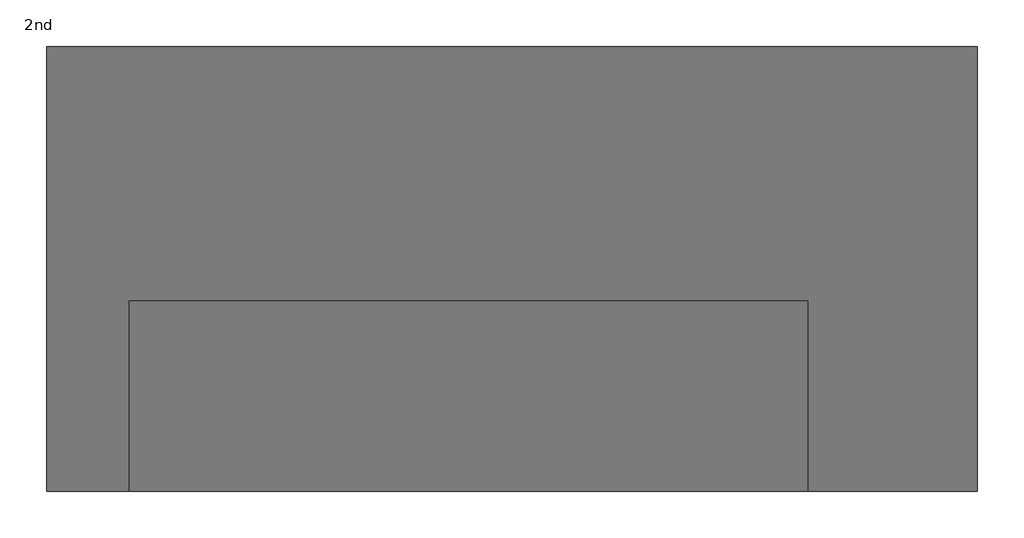
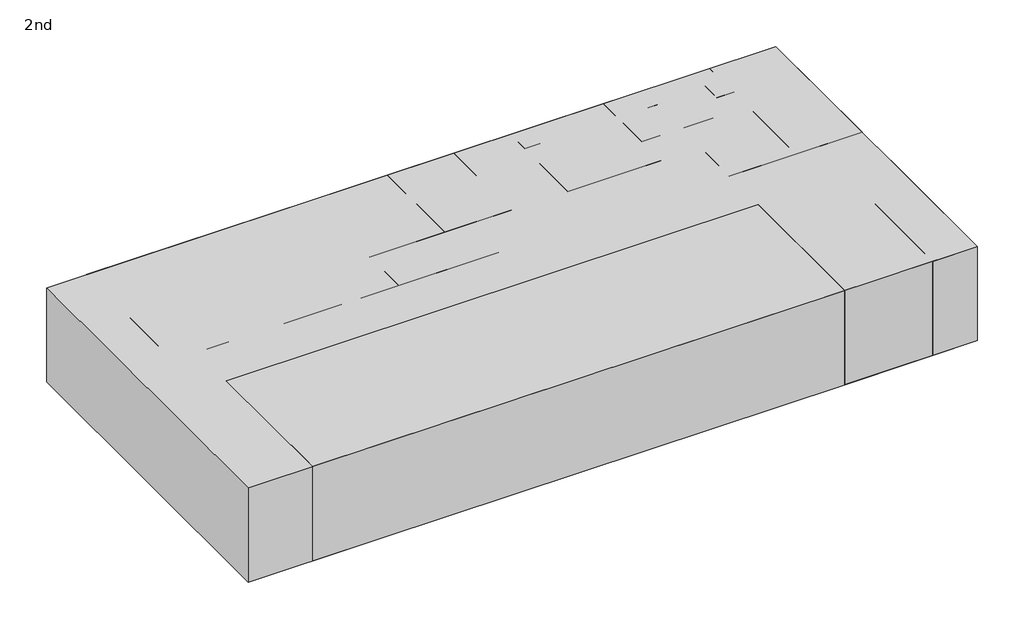
# One storey: 17 proxies.
"""IFC4 building model written with IfcOpenShell, lengths in millimetres."""

import ifcopenshell
import ifcopenshell.guid

model = None  # the IFC model being written
_history = None  # IfcOwnerHistory: only IFC2X3 demands one
_inside = {}  # id of a spatial element -> (the spatial element, [elements in it])
_under = {}  # id of a project, library or spatial element -> (it, [spatial elements below it])
_declared = {}  # id of a project -> (the project, [libraries it declares])
_typed = {}  # id of a type object -> (the type object, [elements of that type])
_made_of = {}  # id of a material, layer set ... -> (it, [elements and type objects made of it])


def new_model(schema):
    """Start an empty IFC model of exactly this schema.

    Asked for "IFC4X3", IfcOpenShell would pick the latest addendum, in which some entities
    have other attributes; the version numbers below select the first issue.
    IFC2X3 requires an IfcOwnerHistory on every rooted entity: one is made here for all.
    """
    global model, _history
    if schema == "IFC4X3":
        model = ifcopenshell.file(schema_version=(4, 3, 0, 0))
    else:
        model = ifcopenshell.file(schema=schema)
    _inside.clear()
    _under.clear()
    _declared.clear()
    _typed.clear()
    _made_of.clear()
    _history = None
    if model.schema == "IFC2X3":
        org = make("IfcOrganization", Name="unknown")
        user = make(
            "IfcPersonAndOrganization",
            ThePerson=make("IfcPerson", FamilyName="unknown"),
            TheOrganization=org,
        )
        app = make(
            "IfcApplication",
            ApplicationDeveloper=org,
            Version="unknown",
            ApplicationFullName="unknown",
            ApplicationIdentifier="unknown",
        )
        _history = make(
            "IfcOwnerHistory",
            OwningUser=user,
            OwningApplication=app,
            ChangeAction="ADDED",
            CreationDate=0,
        )
    return model


def make(cls, **values):
    """One entity of the class cls with the attributes given. An attribute that is None is left unset."""
    return model.create_entity(
        cls, **{name: value for name, value in values.items() if value is not None}
    )


def rooted(cls, **values):
    """An entity with a GlobalId (a new one), such as an element, a storey or a relation."""
    return make(cls, GlobalId=ifcopenshell.guid.new(), OwnerHistory=_history, **values)


def si_unit(unit_type, name, prefix=None):
    """IfcSIUnit, for example si_unit("LENGTHUNIT", "METRE", prefix="MILLI")."""
    return make("IfcSIUnit", UnitType=unit_type, Prefix=prefix, Name=name)


def assignment(units):
    """IfcUnitAssignment: the units of a project."""
    return None if units is None else make("IfcUnitAssignment", Units=units)


def point(xyz):
    """IfcCartesianPoint."""
    return None if xyz is None else make("IfcCartesianPoint", Coordinates=xyz)


def direction(xyz):
    """IfcDirection."""
    return None if xyz is None else make("IfcDirection", DirectionRatios=xyz)


def frame(location, z_axis=None, x_axis=None):
    """IfcAxis2Placement3D, a coordinate frame: its origin and axes. An axis left out is left unset."""
    return make(
        "IfcAxis2Placement3D",
        Location=point(location),
        Axis=direction(z_axis),
        RefDirection=direction(x_axis),
    )


def origin():
    """The frame at (0, 0, 0) with its axes left unset."""
    return frame((0.0, 0.0, 0.0))


def origin_with_axes():
    """The frame at (0, 0, 0) with the z axis (0, 0, 1) and the x axis (1, 0, 0) written out."""
    return frame((0.0, 0.0, 0.0), z_axis=(0.0, 0.0, 1.0), x_axis=(1.0, 0.0, 0.0))


def place(relative_to, where):
    """IfcLocalPlacement: puts the frame where relative to a parent placement (None: the world)."""
    return make(
        "IfcLocalPlacement", PlacementRelTo=relative_to, RelativePlacement=where
    )


def context(
    kind, dimensions, precision=None, world=None, true_north=None, identifier=None
):
    """IfcGeometricRepresentationContext, for example the 3D "Model" context."""
    return make(
        "IfcGeometricRepresentationContext",
        ContextIdentifier=identifier,
        ContextType=kind,
        CoordinateSpaceDimension=dimensions,
        Precision=precision,
        WorldCoordinateSystem=world,
        TrueNorth=true_north,
    )


def project(units=None, contexts=None):
    """IfcProject with its units and contexts."""
    return rooted(
        "IfcProject",
        Name="project",
        RepresentationContexts=contexts,
        UnitsInContext=assignment(units),
    )


def spatial(cls, under=None, at=None, **own):
    """A site, building, storey or space (cls), placed at a placement, below another one or the project."""
    s = rooted(cls, ObjectPlacement=at, **own)
    if under is not None:
        _under.setdefault(under.id(), (under, []))[1].append(s)
    return s


def polyline(points):
    """IfcPolyline through the points."""
    return make("IfcPolyline", Points=[point(p) for p in points])


def outline(outer, holes=None, kind="AREA"):
    """IfcArbitraryClosedProfileDef: a profile drawn as a closed curve; with holes, ...WithVoids."""
    if holes is None:
        return make("IfcArbitraryClosedProfileDef", ProfileType=kind, OuterCurve=outer)
    return make(
        "IfcArbitraryProfileDefWithVoids",
        ProfileType=kind,
        OuterCurve=outer,
        InnerCurves=holes,
    )


def extrude(swept, where, along, depth):
    """IfcExtrudedAreaSolid: the profile swept, set in the frame where, extruded along a direction by depth."""
    return make(
        "IfcExtrudedAreaSolid",
        SweptArea=swept,
        Position=where,
        ExtrudedDirection=direction(along),
        Depth=depth,
    )


def shape(context_of_items, identifier, shape_type, items):
    """IfcShapeRepresentation: the items that make up one representation, for example the "Body"."""
    return make(
        "IfcShapeRepresentation",
        ContextOfItems=context_of_items,
        RepresentationIdentifier=identifier,
        RepresentationType=shape_type,
        Items=items,
    )


def source(mapping_origin, context_of_items, identifier, shape_type, items):
    """IfcRepresentationMap: a shape defined once, which mapped items show again and again."""
    return make(
        "IfcRepresentationMap",
        MappingOrigin=mapping_origin,
        MappedRepresentation=shape(context_of_items, identifier, shape_type, items),
    )


def transform(
    local_origin,
    x_axis=None,
    y_axis=None,
    z_axis=None,
    scale=None,
    scale2=None,
    scale3=None,
    uniform=True,
):
    """IfcCartesianTransformationOperator3D, or its non-uniform kind. x_axis, y_axis, z_axis: its Axis1, 2, 3."""
    if uniform:
        return make(
            "IfcCartesianTransformationOperator3D",
            Axis1=direction(x_axis),
            Axis2=direction(y_axis),
            LocalOrigin=point(local_origin),
            Scale=scale,
            Axis3=direction(z_axis),
        )
    return make(
        "IfcCartesianTransformationOperator3DnonUniform",
        Axis1=direction(x_axis),
        Axis2=direction(y_axis),
        LocalOrigin=point(local_origin),
        Scale=scale,
        Axis3=direction(z_axis),
        Scale2=scale2,
        Scale3=scale3,
    )


def mapped(mapping_source, mapping_target):
    """IfcMappedItem: shows the shape of a source again, moved by a transform."""
    return make(
        "IfcMappedItem", MappingSource=mapping_source, MappingTarget=mapping_target
    )


def made_of(thing, what):
    """Note that an element or type object is made of a material, layer set ...; save() writes the relation."""
    if what is not None:
        _made_of.setdefault(what.id(), (what, []))[1].append(thing)
    return thing


def element(
    cls,
    number,
    at=None,
    inside=None,
    cuts=None,
    type_object=None,
    material=None,
    context=None,
    identifier="Body",
    shape_type=None,
    held_by="IfcProductDefinitionShape",
    body=None,
    shapes=None,
    **own,
):
    """One element of the class cls, such as IfcWall. Its Tag is "e" and its number.

    at: its placement. inside: the storey or other place that contains it. cuts: it is an
    opening in that element (IfcRelVoidsElement). A single representation is given by context,
    identifier, shape_type and body (its items); several are given by shapes. held_by: the class
    of the entity that holds the representations. save() writes the other relations.
    """
    e = rooted(cls, Tag="e%d" % number, ObjectPlacement=at, **own)
    if body is not None:
        shapes = [shape(context, identifier, shape_type, body)]
    if shapes is not None:
        e.Representation = make(held_by, Representations=shapes)
    if inside is not None:
        _inside.setdefault(inside.id(), (inside, []))[1].append(e)
    if cuts is not None:
        rooted(
            "IfcRelVoidsElement", RelatingBuildingElement=cuts, RelatedOpeningElement=e
        )
    if type_object is not None:
        _typed.setdefault(type_object.id(), (type_object, []))[1].append(e)
    return made_of(e, material)


def aggregate(whole, parts):
    """IfcRelAggregates: a whole, such as a stair, and the parts it consists of."""
    return rooted("IfcRelAggregates", RelatingObject=whole, RelatedObjects=parts)


def save(model, path):
    """Write the relations noted so far, then the file.

    IfcRelAggregates (storeys below a building ...), IfcRelContainedInSpatialStructure (elements
    in a storey), IfcRelDefinesByType, IfcRelAssociatesMaterial and IfcRelDeclares: one each for
    every whole, place, type object, material and project.
    """
    for whole, parts in _under.values():
        aggregate(whole, parts)
    for where, things in _inside.values():
        rooted(
            "IfcRelContainedInSpatialStructure",
            RelatedElements=things,
            RelatingStructure=where,
        )
    for kind, things in _typed.values():
        rooted("IfcRelDefinesByType", RelatedObjects=things, RelatingType=kind)
    for what, things in _made_of.values():
        rooted("IfcRelAssociatesMaterial", RelatedObjects=things, RelatingMaterial=what)
    for by, libraries in _declared.values():
        rooted("IfcRelDeclares", RelatingContext=by, RelatedDefinitions=libraries)
    model.write(path)


def generic_models_29bcd6f9(model_context):
    return source(origin(), model_context, "Body", "SweptSolid", [
        extrude(outline(polyline([(2000.0, 4500.0), (2000.0, -4500.0), (-2000.0, -4500.0), (-2000.0, 4500.0), (2000.0, 4500.0)])), origin_with_axes(), (0.0, 0.0, 1.0), 6000.0),
    ])


def generic_models_5634f436(model_context):
    return source(origin(), model_context, "Body", "SweptSolid", [
        extrude(outline(polyline([(1350.0, 3000.0), (1350.0, -3000.0), (-1350.0, -3000.0), (-1350.0, 3000.0), (1350.0, 3000.0)])), origin_with_axes(), (0.0, 0.0, 1.0), 6000.0),
    ])


def generic_models_71e2440f(model_context):
    return source(origin(), model_context, "Body", "SweptSolid", [
        extrude(outline(polyline([(500.0, 1250.0), (500.0, -1250.0), (-500.0, -1250.0), (-500.0, 1250.0), (500.0, 1250.0)])), origin_with_axes(), (0.0, 0.0, 1.0), 6000.0),
    ])


def generic_models_57c7875f(model_context):
    return source(origin(), model_context, "Body", "SweptSolid", [
        extrude(outline(polyline([(4500.0, 16000.0), (4500.0, -16000.0), (-4500.0, -16000.0), (-4500.0, 16000.0), (4500.0, 16000.0)])), origin_with_axes(), (0.0, 0.0, 1.0), 6000.0),
    ])


def generic_models_7bff30ad(model_context):
    return source(origin(), model_context, "Body", "SweptSolid", [
        extrude(outline(polyline([(2000.0, 2000.0), (2000.0, -2000.0), (-2000.0, -2000.0), (-2000.0, 2000.0), (2000.0, 2000.0)])), origin_with_axes(), (0.0, 0.0, 1.0), 6000.0),
    ])


def generic_models_5b7b272c(model_context):
    return source(origin(), model_context, "Body", "SweptSolid", [
        extrude(outline(polyline([(2000.0, 2500.0), (2000.0, -2500.0), (-2000.0, -2500.0), (-2000.0, 2500.0), (2000.0, 2500.0)])), origin_with_axes(), (0.0, 0.0, 1.0), 6000.0),
    ])


def generic_models_47b98be1(model_context):
    return source(origin(), model_context, "Body", "SweptSolid", [
        extrude(outline(polyline([(1200.0, 2000.0), (1200.0, -2000.0), (-1200.0, -2000.0), (-1200.0, 2000.0), (1200.0, 2000.0)])), origin_with_axes(), (0.0, 0.0, 1.0), 6000.0),
    ])


def generic_models_7a053eeb(model_context):
    return source(origin(), model_context, "Body", "SweptSolid", [
        extrude(outline(polyline([(1200.0, 750.0), (1200.0, -750.0), (-1200.0, -750.0), (-1200.0, 750.0), (1200.0, 750.0)])), origin_with_axes(), (0.0, 0.0, 1.0), 6000.0),
    ])


def generic_models_ec17d728(model_context):
    return source(origin(), model_context, "Body", "SweptSolid", [
        extrude(outline(polyline([(2800.0, 3000.0), (2800.0, -3000.0), (-2800.0, -3000.0), (-2800.0, 3000.0), (2800.0, 3000.0)])), origin_with_axes(), (0.0, 0.0, 1.0), 6000.0),
    ])


def generic_models_85897e09(model_context):
    return source(origin(), model_context, "Body", "SweptSolid", [
        extrude(outline(polyline([(2800.0, 750.0), (2800.0, -750.0), (-2800.0, -750.0), (-2800.0, 750.0), (2800.0, 750.0)])), origin_with_axes(), (0.0, 0.0, 1.0), 6000.0),
    ])


def generic_models_b79df083(model_context):
    return source(origin(), model_context, "Body", "SweptSolid", [
        extrude(outline(polyline([(4500.0, 4500.0), (4500.0, -4500.0), (-4500.0, -4500.0), (-4500.0, 4500.0), (4500.0, 4500.0)])), origin_with_axes(), (0.0, 0.0, 1.0), 6000.0),
    ])


def generic_models_98b71764(model_context):
    return source(origin(), model_context, "Body", "SweptSolid", [
        extrude(outline(polyline([(2000.0, 3000.0), (2000.0, -3000.0), (-2000.0, -3000.0), (-2000.0, 3000.0), (2000.0, 3000.0)])), origin_with_axes(), (0.0, 0.0, 1.0), 6000.0),
    ])


def generic_models_8af91fed(model_context):
    return source(origin(), model_context, "Body", "SweptSolid", [
        extrude(outline(polyline([(2250.0, 3000.0), (2250.0, -3000.0), (-2250.0, -3000.0), (-2250.0, 3000.0), (2250.0, 3000.0)])), origin_with_axes(), (0.0, 0.0, 1.0), 6000.0),
    ])


def generic_models_542cc789(model_context):
    return source(origin(), model_context, "Body", "SweptSolid", [
        extrude(outline(polyline([(1500.0, 3000.0), (1500.0, -3000.0), (-1500.0, -3000.0), (-1500.0, 3000.0), (1500.0, 3000.0)])), origin_with_axes(), (0.0, 0.0, 1.0), 6000.0),
    ])


def generic_models_af0009da(model_context):
    return source(origin(), model_context, "Body", "SweptSolid", [
        extrude(outline(polyline([(4500.0, 6800.0), (4500.0, -6800.0), (-4500.0, -6800.0), (-4500.0, 6800.0), (4500.0, 6800.0)])), origin_with_axes(), (0.0, 0.0, 1.0), 6000.0),
    ])


def generic_models_4d084078(model_context):
    return source(origin(), model_context, "Body", "SweptSolid", [
        extrude(outline(polyline([(4000.0, 4500.0), (4000.0, -4500.0), (-4000.0, -4500.0), (-4000.0, 4500.0), (4000.0, 4500.0)])), origin_with_axes(), (0.0, 0.0, 1.0), 6000.0),
    ])


def generic_models_b3b0fa1d(model_context):
    return source(origin(), model_context, "Body", "SweptSolid", [
        extrude(outline(polyline([(21950.0, 10500.0), (21950.0, -10500.0), (-21950.0, -10500.0), (-21950.0, 10500.0), (21950.0, 10500.0)])), origin_with_axes(), (0.0, 0.0, 1.0), 6000.0),
    ])


model = new_model("IFC4")

# Units and contexts
model_context = context("Model", 3, world=origin())
ifc_project = project(units=[si_unit("LENGTHUNIT", "METRE", prefix="MILLI")], contexts=[model_context])

# Site, building, storey
site = spatial("IfcSite", under=ifc_project)
building = spatial("IfcBuilding", under=site)
storey = spatial("IfcBuildingStorey", under=building, Name="2nd", Elevation=14000.0)

# Proxies
placement = place(None, origin())
generic_models_shape = generic_models_29bcd6f9(model_context)
element("IfcBuildingElementProxy", 1, Name="Space Planning Box_hec : Space Planning Box_hec", ObjectType="Space Planning Box_hec : Space Planning Box_hec", at=placement, inside=storey, context=model_context, shape_type="MappedRepresentation", body=[
    mapped(generic_models_shape, transform((198014.1020501, 147515.7581198, 14000.0), x_axis=(1.0, 0.0, 0.0), y_axis=(0.0, 1.0, 0.0), z_axis=(0.0, 0.0, 1.0))),
])
generic_models_2_shape = generic_models_5634f436(model_context)
element("IfcBuildingElementProxy", 2, Name="Space Planning Box_hec : Space Planning Box_hec", ObjectType="Space Planning Box_hec : Space Planning Box_hec", at=placement, inside=storey, context=model_context, shape_type="MappedRepresentation", body=[
    mapped(generic_models_2_shape, transform((198664.1020501, 134015.7581198, 14000.0), x_axis=(1.0, 0.0, 0.0), y_axis=(0.0, 1.0, 0.0), z_axis=(0.0, 0.0, 1.0))),
])
generic_models_3_shape = generic_models_71e2440f(model_context)
element("IfcBuildingElementProxy", 3, Name="Space Planning Box_hec : Space Planning Box_hec", ObjectType="Space Planning Box_hec : Space Planning Box_hec", at=placement, inside=storey, context=model_context, shape_type="MappedRepresentation", body=[
    mapped(generic_models_3_shape, transform((195514.1020501, 150765.7581198, 14000.0), x_axis=(1.0, 0.0, 0.0), y_axis=(0.0, 1.0, 0.0), z_axis=(0.0, 0.0, 1.0))),
])
generic_models_4_shape = generic_models_57c7875f(model_context)
element("IfcBuildingElementProxy", 4, Name="Space Planning Box_hec : Space Planning Box_hec", ObjectType="Space Planning Box_hec : Space Planning Box_hec", at=placement, inside=storey, context=model_context, shape_type="MappedRepresentation", body=[
    mapped(generic_models_4_shape, transform((176014.1020501, 135515.7581198, 14000.0), x_axis=(0.0, -1.0, 0.0), y_axis=(1.0, 0.0, 0.0), z_axis=(0.0, 0.0, 1.0))),
])
generic_models_5_shape = generic_models_7bff30ad(model_context)
element("IfcBuildingElementProxy", 5, Name="Space Planning Box_hec : Space Planning Box_hec", ObjectType="Space Planning Box_hec : Space Planning Box_hec", at=placement, inside=storey, context=model_context, shape_type="MappedRepresentation", body=[
    mapped(generic_models_5_shape, transform((194014.1020501, 150015.7581198, 14000.0), x_axis=(1.0, 0.0, 0.0), y_axis=(0.0, 1.0, 0.0), z_axis=(0.0, 0.0, 1.0))),
])
generic_models_6_shape = generic_models_5b7b272c(model_context)
element("IfcBuildingElementProxy", 6, Name="Space Planning Box_hec : Space Planning Box_hec", ObjectType="Space Planning Box_hec : Space Planning Box_hec", at=placement, inside=storey, context=model_context, shape_type="MappedRepresentation", body=[
    mapped(generic_models_6_shape, transform((194014.1020501, 145515.7581198, 14000.0), x_axis=(1.0, 0.0, 0.0), y_axis=(0.0, 1.0, 0.0), z_axis=(0.0, 0.0, 1.0))),
])
generic_models_7_shape = generic_models_47b98be1(model_context)
element("IfcBuildingElementProxy", 7, Name="Space Planning Box_hec : Space Planning Box_hec", ObjectType="Space Planning Box_hec : Space Planning Box_hec", at=placement, inside=storey, context=model_context, shape_type="MappedRepresentation", body=[
    mapped(generic_models_7_shape, transform((190814.1020501, 150015.7581198, 14000.0), x_axis=(1.0, 0.0, 0.0), y_axis=(0.0, 1.0, 0.0), z_axis=(0.0, 0.0, 1.0))),
])
generic_models_8_shape = generic_models_7a053eeb(model_context)
element("IfcBuildingElementProxy", 8, Name="Space Planning Box_hec : Space Planning Box_hec", ObjectType="Space Planning Box_hec : Space Planning Box_hec", at=placement, inside=storey, context=model_context, shape_type="MappedRepresentation", body=[
    mapped(generic_models_8_shape, transform((190814.1020501, 151265.7581198, 14000.0), x_axis=(1.0, 0.0, 0.0), y_axis=(0.0, 1.0, 0.0), z_axis=(0.0, 0.0, 1.0))),
])
generic_models_9_shape = generic_models_ec17d728(model_context)
element("IfcBuildingElementProxy", 9, Name="Space Planning Box_hec : Space Planning Box_hec", ObjectType="Space Planning Box_hec : Space Planning Box_hec", at=placement, inside=storey, context=model_context, shape_type="MappedRepresentation", body=[
    mapped(generic_models_9_shape, transform((186814.1020501, 149015.7581198, 14000.0), x_axis=(1.0, 0.0, 0.0), y_axis=(0.0, 1.0, 0.0), z_axis=(0.0, 0.0, 1.0))),
])
generic_models_10_shape = generic_models_85897e09(model_context)
element("IfcBuildingElementProxy", 10, Name="Space Planning Box_hec : Space Planning Box_hec", ObjectType="Space Planning Box_hec : Space Planning Box_hec", at=placement, inside=storey, context=model_context, shape_type="MappedRepresentation", body=[
    mapped(generic_models_10_shape, transform((186814.1020501, 151265.7581198, 14000.0), x_axis=(1.0, 0.0, 0.0), y_axis=(0.0, 1.0, 0.0), z_axis=(0.0, 0.0, 1.0))),
])
generic_models_11_shape = generic_models_b79df083(model_context)
element("IfcBuildingElementProxy", 11, Name="Space Planning Box_hec : Space Planning Box_hec", ObjectType="Space Planning Box_hec : Space Planning Box_hec", at=placement, inside=storey, context=model_context, shape_type="MappedRepresentation", body=[
    mapped(generic_models_11_shape, transform((185114.1020501, 147515.7581198, 14000.0), x_axis=(1.0, 0.0, 0.0), y_axis=(0.0, 1.0, 0.0), z_axis=(0.0, 0.0, 1.0))),
])
generic_models_12_shape = generic_models_98b71764(model_context)
element("IfcBuildingElementProxy", 12, Name="Space Planning Box_hec : Space Planning Box_hec", ObjectType="Space Planning Box_hec : Space Planning Box_hec", at=placement, inside=storey, context=model_context, shape_type="MappedRepresentation", body=[
    mapped(generic_models_12_shape, transform((178614.1020501, 149015.7581198, 14000.0), x_axis=(1.0, 0.0, 0.0), y_axis=(0.0, 1.0, 0.0), z_axis=(0.0, 0.0, 1.0))),
])
generic_models_13_shape = generic_models_8af91fed(model_context)
element("IfcBuildingElementProxy", 13, Name="Space Planning Box_hec : Space Planning Box_hec", ObjectType="Space Planning Box_hec : Space Planning Box_hec", at=placement, inside=storey, context=model_context, shape_type="MappedRepresentation", body=[
    mapped(generic_models_13_shape, transform((174364.1020501, 149015.7581198, 14000.0), x_axis=(1.0, 0.0, 0.0), y_axis=(0.0, 1.0, 0.0), z_axis=(0.0, 0.0, 1.0))),
])
generic_models_14_shape = generic_models_542cc789(model_context)
element("IfcBuildingElementProxy", 14, Name="Space Planning Box_hec : Space Planning Box_hec", ObjectType="Space Planning Box_hec : Space Planning Box_hec", at=placement, inside=storey, context=model_context, shape_type="MappedRepresentation", body=[
    mapped(generic_models_14_shape, transform((175114.1020501, 144515.7581198, 14000.0), x_axis=(0.0, 1.0, 0.0), y_axis=(-1.0, 0.0, 0.0), z_axis=(0.0, 0.0, 1.0))),
])
generic_models_15_shape = generic_models_af0009da(model_context)
element("IfcBuildingElementProxy", 15, Name="Space Planning Box_hec : Space Planning Box_hec", ObjectType="Space Planning Box_hec : Space Planning Box_hec", at=placement, inside=storey, context=model_context, shape_type="MappedRepresentation", body=[
    mapped(generic_models_15_shape, transform((165314.1020501, 147515.7581198, 14000.0), x_axis=(0.0, -1.0, 0.0), y_axis=(1.0, 0.0, 0.0), z_axis=(0.0, 0.0, 1.0))),
])
generic_models_16_shape = generic_models_4d084078(model_context)
element("IfcBuildingElementProxy", 16, Name="Space Planning Box_hec : Space Planning Box_hec", ObjectType="Space Planning Box_hec : Space Planning Box_hec", at=placement, inside=storey, context=model_context, shape_type="MappedRepresentation", body=[
    mapped(generic_models_16_shape, transform((196014.1020501, 135515.7581198, 14000.0), x_axis=(1.0, 0.0, 0.0), y_axis=(0.0, 1.0, 0.0), z_axis=(0.0, 0.0, 1.0))),
])
generic_models_17_shape = generic_models_b3b0fa1d(model_context)
element("IfcBuildingElementProxy", 17, Name="Space Planning Box_hec : Space Planning Box_hec", ObjectType="Space Planning Box_hec : Space Planning Box_hec", at=placement, inside=storey, context=model_context, shape_type="MappedRepresentation", body=[
    mapped(generic_models_17_shape, transform((178064.1020501, 141515.7581198, 14000.0), x_axis=(1.0, 0.0, 0.0), y_axis=(0.0, 1.0, 0.0), z_axis=(0.0, 0.0, 1.0))),
])

save(model, "model.ifc")

# Revit data of these elements
# Type "Space Planning Box_hec : Space Planning Box_hec"
#   Type Comments = "..."
#   Room Name [instance default] = "?"
#   Interior Finish [instance default] = ""
#   Exterior Finish [instance default] = ""
#   Department [instance default] = ""
#   Assembly Code = "..."
#   Width [instance default] = 1524 mm
#   Program Area [instance default] = 0 m²
#   Length [instance default] = 1524 mm
#   Height [instance default] = 1524 mm
#   Area [instance default] = 2.32258 m²
#   Fill Color [instance default] = Cyan
#   Default Elevation = 0
# Element 1 (IfcBuildingElementProxy, "Space Planning Box_hec : Space Planning Box_hec")
#   Room Name = "Stairway"
#   Interior Finish = "IF2"
#   Exterior Finish = "EF1"
#   Department = "AR"
#   Width = 4000 mm
#   Program Area = 38 m²
#   Length = 9000 mm
#   Height = 6000 mm
#   Area = 36 m²
#   Fill Color = Lavender
#   Phase Created = New Construction
#   Materials on its faces: "Lavender"
# Element 2 (IfcBuildingElementProxy, "Space Planning Box_hec : Space Planning Box_hec")
#   Room Name = "Duct Shaft"
#   Interior Finish = "NA"
#   Exterior Finish = "EF1"
#   Department = "HV"
#   Width = 2700 mm
#   Program Area = 16.2 m²
#   Length = 6000 mm
#   Height = 6000 mm
#   Area = 16.2 m²
#   Fill Color = Pink
#   Phase Created = New Construction
#   Materials on its faces: "Pink"
# Element 3 (IfcBuildingElementProxy, "Space Planning Box_hec : Space Planning Box_hec")
#   Room Name = "Pipe Shaft"
#   Interior Finish = "NA"
#   Exterior Finish = "EF1"
#   Department = "HV"
#   Width = 1000 mm
#   Program Area = 2.5 m²
#   Length = 2500 mm
#   Height = 6000 mm
#   Area = 2.5 m²
#   Fill Color = Pink
#   Phase Created = New Construction
#   Materials on its faces: "Pink"
# Element 4 (IfcBuildingElementProxy, "Space Planning Box_hec : Space Planning Box_hec")
#   Room Name = "Central Control Room"
#   Interior Finish = "IF3"
#   Exterior Finish = "EF1"
#   Department = "CI"
#   Width = 9000 mm
#   Program Area = 288 m²
#   Length = 32000 mm
#   Height = 6000 mm
#   Area = 288 m²
#   Fill Color = Lime
#   Phase Created = New Construction
#   Materials on its faces: "Lime"
# Element 5 (IfcBuildingElementProxy, "Space Planning Box_hec : Space Planning Box_hec")
#   Room Name = "Toilet (F)"
#   Interior Finish = "IF5"
#   Exterior Finish = "EF1"
#   Department = "AR"
#   Width = 4000 mm
#   Program Area = 72 m²
#   Length = 4000 mm
#   Height = 6000 mm
#   Area = 16 m²
#   Fill Color = Lavender
#   Phase Created = New Construction
#   Materials on its faces: "Lavender"
# Element 6 (IfcBuildingElementProxy, "Space Planning Box_hec : Space Planning Box_hec")
#   Room Name = "Toilet (M)"
#   Interior Finish = "IF5"
#   Exterior Finish = "EF1"
#   Department = "AR"
#   Width = 4000 mm
#   Program Area = 72 m²
#   Length = 5000 mm
#   Height = 6000 mm
#   Area = 20 m²
#   Fill Color = Lavender
#   Phase Created = New Construction
#   Materials on its faces: "Lavender"
# Element 7 (IfcBuildingElementProxy, "Space Planning Box_hec : Space Planning Box_hec")
#   Room Name = "Locker Room (F)"
#   Interior Finish = "IF2-1"
#   Exterior Finish = "EF1"
#   Department = "AR"
#   Width = 2400 mm
#   Program Area = 31.5 m²
#   Length = 4000 mm
#   Height = 6000 mm
#   Area = 9.6 m²
#   Fill Color = Lavender
#   Phase Created = New Construction
#   Materials on its faces: "Lavender"
# Element 8 (IfcBuildingElementProxy, "Space Planning Box_hec : Space Planning Box_hec")
#   Room Name = "Shower Room (F)"
#   Interior Finish = "IF5"
#   Exterior Finish = "EF1"
#   Department = "AR"
#   Width = 2400 mm
#   Program Area = 31.5 m²
#   Length = 1500 mm
#   Height = 6000 mm
#   Area = 3.6 m²
#   Fill Color = Lavender
#   Phase Created = New Construction
#   Materials on its faces: "Lavender"
# Element 9 (IfcBuildingElementProxy, "Space Planning Box_hec : Space Planning Box_hec")
#   Room Name = "Locker Room (M)"
#   Interior Finish = "IF2-1"
#   Exterior Finish = "EF1"
#   Department = "AR"
#   Width = 5600 mm
#   Program Area = 31.5 m²
#   Length = 6000 mm
#   Height = 6000 mm
#   Area = 33.6 m²
#   Fill Color = Lavender
#   Phase Created = New Construction
#   Materials on its faces: "Lavender"
# Element 10 (IfcBuildingElementProxy, "Space Planning Box_hec : Space Planning Box_hec")
#   Room Name = "Shower Room (M)"
#   Interior Finish = "IF5"
#   Exterior Finish = "EF1"
#   Department = "AR"
#   Width = 5600 mm
#   Program Area = 31.5 m²
#   Length = 1500 mm
#   Height = 6000 mm
#   Area = 8.4 m²
#   Fill Color = Lavender
#   Phase Created = New Construction
#   Materials on its faces: "Lavender"
# Element 11 (IfcBuildingElementProxy, "Space Planning Box_hec : Space Planning Box_hec")
#   Room Name = "Kitch & Lunch Room"
#   Interior Finish = "IF2-1"
#   Exterior Finish = "EF1"
#   Department = "AR"
#   Width = 9000 mm
#   Program Area = 31.5 m²
#   Length = 9000 mm
#   Height = 6000 mm
#   Area = 81 m²
#   Fill Color = Lavender
#   Phase Created = New Construction
#   Materials on its faces: "Lavender"
# Element 12 (IfcBuildingElementProxy, "Space Planning Box_hec : Space Planning Box_hec")
#   Room Name = "Shift Office Room"
#   Interior Finish = "IF2-1"
#   Exterior Finish = "EF1"
#   Department = "AR"
#   Width = 4000 mm
#   Program Area = 43.2 m²
#   Length = 6000 mm
#   Height = 6000 mm
#   Area = 24 m²
#   Fill Color = Lavender
#   Phase Created = New Construction
#   Materials on its faces: "Lavender"
# Element 13 (IfcBuildingElementProxy, "Space Planning Box_hec : Space Planning Box_hec")
#   Room Name = "Document Room"
#   Interior Finish = "IF2-1"
#   Exterior Finish = "EF1"
#   Department = "AR"
#   Width = 4500 mm
#   Program Area = 48 m²
#   Length = 6000 mm
#   Height = 6000 mm
#   Area = 27 m²
#   Fill Color = Lavender
#   Phase Created = New Construction
#   Materials on its faces: "Lavender"
# Element 14 (IfcBuildingElementProxy, "Space Planning Box_hec : Space Planning Box_hec")
#   Room Name = "LOTO Office Room"
#   Interior Finish = "IF2-1"
#   Exterior Finish = "EF1"
#   Department = "AR"
#   Width = 3000 mm
#   Program Area = 31.5 m²
#   Length = 6000 mm
#   Height = 6000 mm
#   Area = 18 m²
#   Fill Color = Lavender
#   Phase Created = New Construction
#   Materials on its faces: "Lavender"
# Element 15 (IfcBuildingElementProxy, "Space Planning Box_hec : Space Planning Box_hec")
#   Room Name = "Engineer Room"
#   Interior Finish = "IF3"
#   Exterior Finish = "EF1"
#   Department = "CI"
#   Width = 9000 mm
#   Program Area = 120 m²
#   Length = 13600 mm
#   Height = 6000 mm
#   Area = 122.4 m²
#   Fill Color = Lime
#   Phase Created = New Construction
#   Materials on its faces: "Lime"
# Element 16 (IfcBuildingElementProxy, "Space Planning Box_hec : Space Planning Box_hec")
#   Room Name = "Fire Gas Room"
#   Interior Finish = "IF1"
#   Exterior Finish = "EF1"
#   Department = "SF"
#   Width = 8000 mm
#   Program Area = 0 m²
#   Length = 9000 mm
#   Height = 6000 mm
#   Area = 72 m²
#   Fill Color = Cyan
#   Phase Created = New Construction
#   Materials on its faces: "Cyan"
# Element 17 (IfcBuildingElementProxy, "Space Planning Box_hec : Space Planning Box_hec")
#   Room Name = "Corridor"
#   Interior Finish = "IF2-1"
#   Exterior Finish = "EF1"
#   Department = "AR"
#   Width = 43900 mm
#   Program Area = 0 m²
#   Length = 21000 mm
#   Height = 6000 mm
#   Area = 921.9 m²
#   Fill Color = Lavender
#   Phase Created = New Construction
#   Materials on its faces: "Lavender"
# Materials
#   "Cyan": class "Generic", colour RGB 0 255 255, transparency 0.2, Cost = 0
#   "Lavender": class "Generic", colour RGB 186 85 211, transparency 0.2, Cost = 0
#   "Pink": class "Generic", colour RGB 255 105 180, transparency 0.2, Cost = 0
#   "Lime": class "Generic", colour RGB 0 255 0, transparency 0.2, Cost = 0
# Room at (190814.102, 151265.758) mm, phase "New Construction", upper offset 2438.4 mm, lower offset 0 mm
#   Number = "3.7"
#   Name = "a"
# Room at (178064.102, 141515.758) mm, phase "New Construction", upper offset 2438.4 mm, lower offset 0 mm
#   Number = "3.8"
#   Name = "a"
# Room at (178614.102, 149015.758) mm, phase "New Construction", upper offset 2438.4 mm, lower offset 0 mm
#   Number = "3.5"
#   Name = "a"
# Room at (175114.102, 144515.758) mm, phase "New Construction", upper offset 2438.4 mm, lower offset 0 mm
#   Number = "3.6"
#   Name = "a"
# Room at (190814.102, 149265.758) mm, phase "New Construction", upper offset 2438.4 mm, lower offset 0 mm
#   Number = "3.9"
#   Name = "a"
# Room at (186814.102, 151265.758) mm, phase "New Construction", upper offset 2438.4 mm, lower offset 0 mm
#   Number = "3.10"
#   Name = "a"
# Room at (185114.102, 145843.189) mm, phase "New Construction", upper offset 2438.4 mm, lower offset 0 mm
#   Number = "3.11"
#   Name = "a"
# Room at (186814.102, 148265.758) mm, phase "New Construction", upper offset 2438.4 mm, lower offset 0 mm
#   Number = "3.12"
#   Name = "a"
# Room at (196014.102, 135515.758) mm, phase "New Construction", upper offset 2438.4 mm, lower offset 0 mm
#   Number = "3.13"
#   Name = "a"
# Room at (198664.102, 134015.758) mm, phase "New Construction", upper offset 2438.4 mm, lower offset 0 mm
#   Number = "3.14"
#   Name = "a"
# Room at (194014.102, 150015.758) mm, phase "New Construction", upper offset 2438.4 mm, lower offset 0 mm
#   Number = "3.15"
#   Name = "a"
# Room at (195514.102, 150765.758) mm, phase "New Construction", upper offset 2438.4 mm, lower offset 0 mm
#   Number = "3.16"
#   Name = "a"
# Room at (176014.102, 135515.758) mm, phase "New Construction", upper offset 2438.4 mm, lower offset 0 mm
#   Number = "3.0"
#   Name = "a"
# Room at (165314.102, 147515.758) mm, phase "New Construction", upper offset 2438.4 mm, lower offset 0 mm
#   Number = "3.1"
#   Name = "a"
# Room at (174364.102, 149015.758) mm, phase "New Construction", upper offset 2438.4 mm, lower offset 0 mm
#   Number = "3.2"
#   Name = "a"
# Room at (194014.102, 145515.758) mm, phase "New Construction", upper offset 2438.4 mm, lower offset 0 mm
#   Number = "3.3"
#   Name = "a"
# Room at (198014.102, 147515.758) mm, phase "New Construction", upper offset 2438.4 mm, lower offset 0 mm
#   Number = "3.4"
#   Name = "a"
